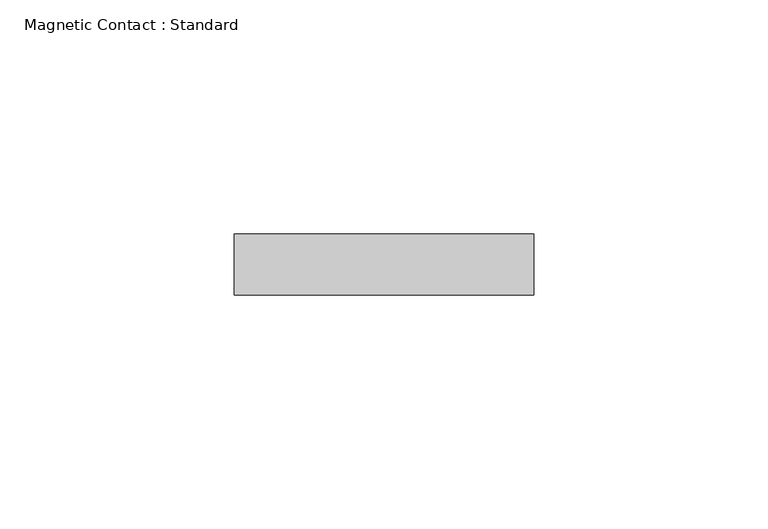
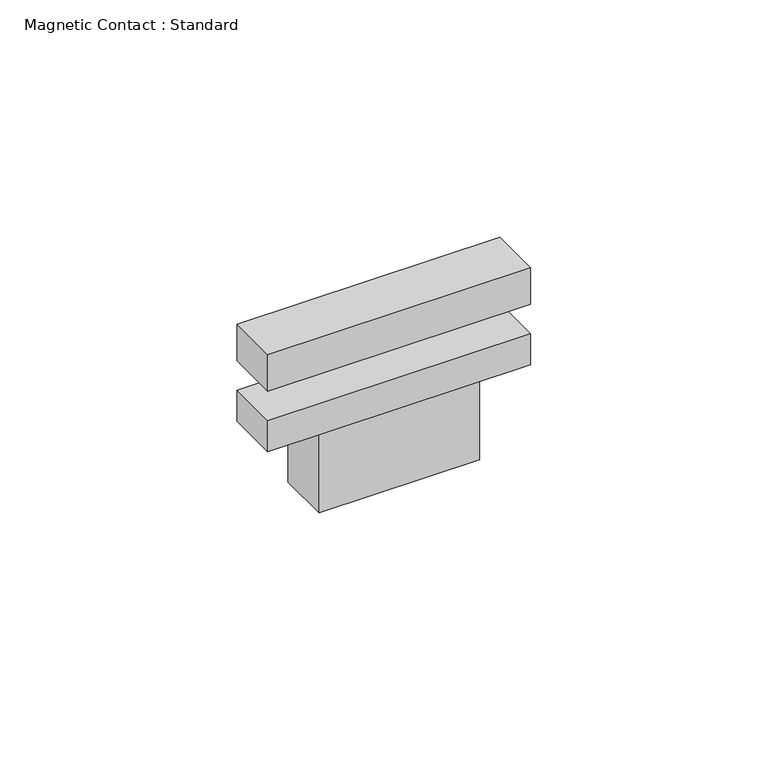
"""IFC4 building model written with IfcOpenShell, lengths in millimetres: proxy geometry, Magnetic Contact : Standard."""

from ifc_helpers import new_model, si_unit, frame, origin, origin_with_axes, place, context, project, spatial, polyline, outline, extrude, source, transform, mapped, element, save


def magnetic_contact_standard_a188dc91(model_context):
    return source(origin(), model_context, "Body", "SweptSolid", [
        extrude(outline(polyline([(32.0, 13.0), (32.0, 0.0), (-32.0, 0.0), (-32.0, 13.0), (32.0, 13.0)])), frame((0.0, 0.0, 15.5767529), z_axis=(0.0, 0.0, 1.0), x_axis=(1.0, 0.0, 0.0)), (0.0, 0.0, 1.0), 9.4232471),
        extrude(outline(polyline([(32.0, 13.0), (32.0, 0.0), (-32.0, 0.0), (-32.0, 13.0), (32.0, 13.0)])), origin_with_axes(), (0.0, 0.0, 1.0), 8.0),
        extrude(outline(polyline([(19.5, 13.0), (19.5, 0.0), (-19.5, 0.0), (-19.5, 13.0), (19.5, 13.0)])), frame((0.0, 0.0, -20.0), z_axis=(0.0, 0.0, 1.0), x_axis=(1.0, 0.0, 0.0)), (0.0, 0.0, 1.0), 20.0),
    ])


if __name__ == "__main__":
    model = new_model("IFC4")
    model_context = context("Model", 3, world=origin())
    ifc_project = project(units=[si_unit("LENGTHUNIT", "METRE", prefix="MILLI")], contexts=[model_context])
    site = spatial("IfcSite", under=ifc_project)
    building = spatial("IfcBuilding", under=site)
    placement = place(None, origin())
    magnetic_contact_standard_shape = magnetic_contact_standard_a188dc91(model_context)
    element("IfcBuildingElementProxy", 1, Name="Magnetic Contact : Standard", ObjectType="Magnetic Contact : Standard", at=placement, inside=building, context=model_context, shape_type="MappedRepresentation", body=[
        mapped(magnetic_contact_standard_shape, transform((0.0, 0.0, 0.0), x_axis=(1.0, 0.0, 0.0), y_axis=(0.0, 1.0, 0.0), z_axis=(0.0, 0.0, 1.0))),
    ])
    save(model, "model.ifc")

# Revit data of these elements
# Type "Magnetic Contact : Standard"
#   Type Mark = "Magnetic Contact"
#   Classification.OmniClass.23.Number = "23-29 11 21"
#   Classification.OmniClass.23.Description = "Security Sensors"
#   COBie.Type.CreatedBy = "info@mma.ie"
#   COBie.Type.CreatedOn = "2017-07-26T09:12:44"
#   COBie.Type.Name = "Magnetic Contact"
#   COBie.Type.Category = "23-29 11 21 : Security Sensors"
#   COBie.Type.Description = "Magnetic Contact_Standard"
#   COBie.Type.AssetType = "Fixed"
#   COBie.Type.Manufacturer = ""
#   COBie.Type.ModelNumber = ""
#   Keynote = "41 24 33.A"
#   COBie.Type.ReplacementCost = 0
#   MC_Width = 64 mm
#   MC_Height = 25 mm
#   MC_Depth = 13 mm
#   Default Elevation = 1200 mm
#   COBie.Type = yes
#   URL = ""
#   Model = ""
#   Manufacturer = ""
